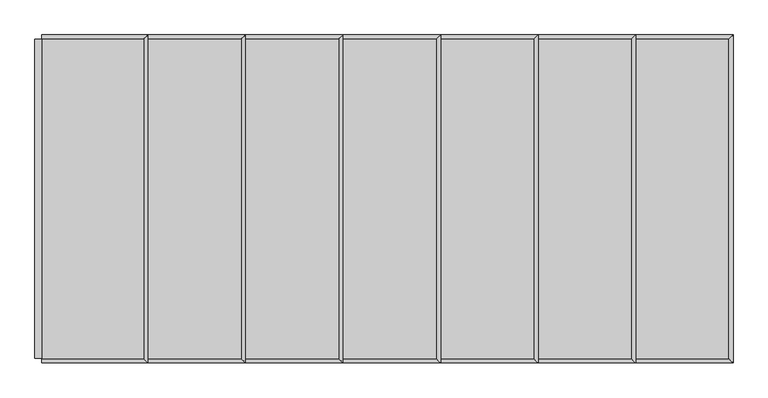
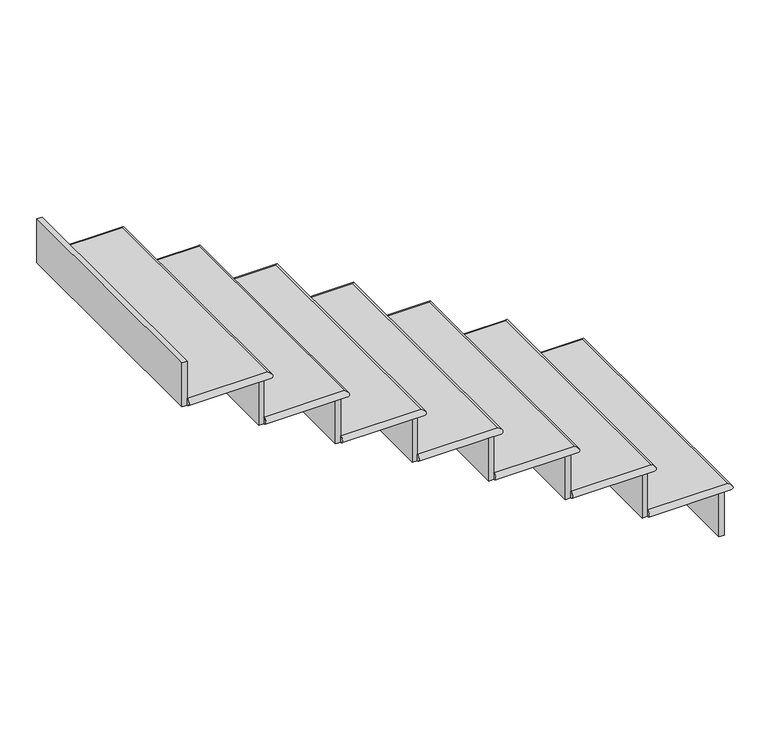
"""IFC4 building model written with IfcOpenShell, lengths in millimetres: stair flight geometry."""

from ifc_helpers import new_model, si_unit, frame, origin, place, context, project, spatial, circle_curve, ellipse_curve, faceted_brep, source, transform, mapped, element, save
from ifc_brep_helpers import plane_surface, cylinder_surface, advanced_brep


def stair_flight_95013a93(model_context):
    return source(origin(), model_context, "Body", "SolidModel", [
        advanced_brep(
        [(-8101.4581077, -7447.633999, 1837.2666667), (-8101.4581077, -7447.633999, 1862.6666667), (-8101.4581077, -8362.033999, 1862.6666667), (-8101.4581077, -8362.033999, 1837.2666667), (-8393.5581077, -7447.633999, 1862.6666667), (-8393.5581077, -8362.033999, 1862.6666667), (-8393.5581077, -8362.033999, 1837.2666667), (-8393.5581077, -7447.633999, 1837.2666667)],
        [
            (0, 1, ellipse_curve(frame((-8101.4581077, -7447.633999, 1849.9666667), z_axis=(0.7071067811865464, -0.7071067811865487, 0.0), x_axis=(0.7071067811865487, 0.7071067811865464, 0.0)), 17.9605122, 12.7)),
            (1, 2),
            (2, 3, ellipse_curve(frame((-8101.4581077, -8362.033999, 1849.9666667), z_axis=(0.7071067811865487, 0.7071067811865464, 0.0), x_axis=(-0.7071067811865464, 0.7071067811865487, 0.0)), 17.9605122, 12.7)),
            (3, 0),
            (4, 5),
            (5, 2),
            (1, 4),
            (6, 7),
            (7, 0),
            (3, 6),
            (4, 7, circle_curve(frame((-8393.5581077, -7447.633999, 1849.9666667), z_axis=(-1.0, 0.0, 0.0), x_axis=(0.0, -1.0, 0.0)), 12.7)),
            (6, 5, circle_curve(frame((-8393.5581077, -8362.033999, 1849.9666667), z_axis=(-1.0, 0.0, 0.0), x_axis=(0.0, 1.0, 0.0)), 12.7)),
        ],
        [
            cylinder_surface(frame((-8101.4581077, -7447.633999, 1849.9666667), z_axis=(0.0, 1.0, 0.0), x_axis=(-1.0, 0.0, 0.0)), 12.7),
            plane_surface(frame((-8088.7581077, -8362.033999, 1862.6666667), z_axis=(0.0, 0.0, 1.0), x_axis=(1.0, 0.0, 0.0))),
            plane_surface(frame((-8088.7581077, -8362.033999, 1837.2666667), z_axis=(0.0, 0.0, -1.0), x_axis=(-1.0, 0.0, 0.0))),
            plane_surface(frame((-8393.5581077, -7447.633999, 1862.6666667), z_axis=(-1.0, 0.0, 0.0), x_axis=(0.0, 0.0, -1.0))),
            cylinder_surface(frame((-8393.5581077, -7447.633999, 1849.9666667), z_axis=(-1.0, 0.0, 0.0), x_axis=(0.0, -1.0, 0.0)), 12.7),
            cylinder_surface(frame((-8101.4581077, -8362.033999, 1849.9666667), z_axis=(1.0, 0.0, 0.0), x_axis=(0.0, 1.0, 0.0)), 12.7),
        ],
        [
            (0, [[1, 2, 3, 4]]),
            (1, [[5, 6, -2, 7]]),
            (2, [[8, 9, -4, 10]]),
            (3, [[-5, 11, -8, 12]]),
            (4, [[-11, -7, -1, -9]]),
            (5, [[-3, -6, -12, -10]]),
        ],
    ),
        faceted_brep([(-8114.1581077, -7447.633999, 1837.2666667), (-8114.1581077, -7447.633999, 1667.9333333), (-8133.2081077, -7447.633999, 1667.9333333), (-8133.2081077, -7447.633999, 1837.2666667), (-8114.1581077, -8362.033999, 1837.2666667), (-8133.2081077, -8362.033999, 1837.2666667), (-8133.2081077, -8362.033999, 1667.9333333), (-8114.1581077, -8362.033999, 1667.9333333)], [[[0, 1, 2, 3]], [[4, 5, 6, 7]], [[1, 0, 4, 7]], [[2, 1, 7, 6]], [[3, 2, 6, 5]], [[0, 3, 5, 4]]]),
        faceted_brep([(-8393.5581077, -7447.633999, 2006.6), (-8393.5581077, -7447.633999, 1837.2666667), (-8412.6081077, -7447.633999, 1837.2666667), (-8412.6081077, -7447.633999, 2006.6), (-8393.5581077, -8362.033999, 2006.6), (-8412.6081077, -8362.033999, 2006.6), (-8412.6081077, -8362.033999, 1837.2666667), (-8393.5581077, -8362.033999, 1837.2666667)], [[[0, 1, 2, 3]], [[4, 5, 6, 7]], [[1, 0, 4, 7]], [[2, 1, 7, 6]], [[3, 2, 6, 5]], [[0, 3, 5, 4]]]),
        advanced_brep(
        [(-8672.9581077, -7447.633999, 2032.0), (-8672.9581077, -8362.033999, 2032.0), (-8380.8581077, -8362.033999, 2032.0), (-8380.8581077, -7447.633999, 2032.0), (-8672.9581077, -8362.033999, 2006.6), (-8672.9581077, -7447.633999, 2006.6), (-8380.8581077, -7447.633999, 2006.6), (-8380.8581077, -8362.033999, 2006.6)],
        [
            (0, 1),
            (1, 2),
            (2, 3),
            (3, 0),
            (4, 5),
            (5, 6),
            (6, 7),
            (7, 4),
            (0, 5, circle_curve(frame((-8672.9581077, -7447.633999, 2019.3), z_axis=(-1.0, 0.0, 0.0), x_axis=(0.0, -1.0, 0.0)), 12.7)),
            (4, 1, circle_curve(frame((-8672.9581077, -8362.033999, 2019.3), z_axis=(-1.0, 0.0, 0.0), x_axis=(0.0, 1.0, 0.0)), 12.7)),
            (6, 3, ellipse_curve(frame((-8380.8581077, -7447.633999, 2019.3), z_axis=(0.707106781186545, -0.7071067811865501, 0.0), x_axis=(0.70710678118655, 0.7071067811865449, 0.0)), 17.9605122, 12.7)),
            (2, 7, ellipse_curve(frame((-8380.8581077, -8362.033999, 2019.3), z_axis=(0.70710678118655, 0.7071067811865449, 0.0), x_axis=(-0.707106781186545, 0.7071067811865501, 0.0)), 17.9605122, 12.7)),
        ],
        [
            plane_surface(frame((-8088.7581077, -8362.033999, 2032.0), z_axis=(0.0, 0.0, 1.0), x_axis=(1.0, 0.0, 0.0))),
            plane_surface(frame((-8088.7581077, -8362.033999, 2006.6), z_axis=(0.0, 0.0, -1.0), x_axis=(-1.0, 0.0, 0.0))),
            plane_surface(frame((-8672.9581077, -7447.633999, 2032.0), z_axis=(-1.0, 0.0, 0.0), x_axis=(0.0, 0.0, -1.0))),
            cylinder_surface(frame((-8380.8581077, -7447.633999, 2019.3), z_axis=(0.0, 1.0, 0.0), x_axis=(-1.0, 0.0, 0.0)), 12.7),
            cylinder_surface(frame((-8672.9581077, -7447.633999, 2019.3), z_axis=(-1.0, 0.0, 0.0), x_axis=(0.0, -1.0, 0.0)), 12.7),
            cylinder_surface(frame((-8380.8581077, -8362.033999, 2019.3), z_axis=(1.0, 0.0, 0.0), x_axis=(0.0, 1.0, 0.0)), 12.7),
        ],
        [
            (0, [[1, 2, 3, 4]]),
            (1, [[5, 6, 7, 8]]),
            (2, [[-1, 9, -5, 10]]),
            (3, [[11, -3, 12, -7]]),
            (4, [[-9, -4, -11, -6]]),
            (5, [[-12, -2, -10, -8]]),
        ],
    ),
        faceted_brep([(-8672.9581077, -7447.633999, 2175.9333333), (-8672.9581077, -7447.633999, 2006.6), (-8692.0081077, -7447.633999, 2006.6), (-8692.0081077, -7447.633999, 2175.9333333), (-8672.9581077, -8362.033999, 2175.9333333), (-8692.0081077, -8362.033999, 2175.9333333), (-8692.0081077, -8362.033999, 2006.6), (-8672.9581077, -8362.033999, 2006.6)], [[[0, 1, 2, 3]], [[4, 5, 6, 7]], [[1, 0, 4, 7]], [[2, 1, 7, 6]], [[3, 2, 6, 5]], [[0, 3, 5, 4]]]),
        advanced_brep(
        [(-8952.3581077, -7447.633999, 2201.3333333), (-8952.3581077, -8362.033999, 2201.3333333), (-8660.2581077, -8362.033999, 2201.3333333), (-8660.2581077, -7447.633999, 2201.3333333), (-8952.3581077, -8362.033999, 2175.9333333), (-8952.3581077, -7447.633999, 2175.9333333), (-8660.2581077, -7447.633999, 2175.9333333), (-8660.2581077, -8362.033999, 2175.9333333)],
        [
            (0, 1),
            (1, 2),
            (2, 3),
            (3, 0),
            (4, 5),
            (5, 6),
            (6, 7),
            (7, 4),
            (0, 5, circle_curve(frame((-8952.3581077, -7447.633999, 2188.6333333), z_axis=(-1.0, 0.0, 0.0), x_axis=(0.0, -1.0, 0.0)), 12.7)),
            (4, 1, circle_curve(frame((-8952.3581077, -8362.033999, 2188.6333333), z_axis=(-1.0, 0.0, 0.0), x_axis=(0.0, 1.0, 0.0)), 12.7)),
            (6, 3, ellipse_curve(frame((-8660.2581077, -7447.633999, 2188.6333333), z_axis=(0.707106781186545, -0.7071067811865501, 0.0), x_axis=(0.70710678118655, 0.7071067811865449, 0.0)), 17.9605122, 12.7)),
            (2, 7, ellipse_curve(frame((-8660.2581077, -8362.033999, 2188.6333333), z_axis=(0.70710678118655, 0.7071067811865449, 0.0), x_axis=(-0.707106781186545, 0.7071067811865501, 0.0)), 17.9605122, 12.7)),
        ],
        [
            plane_surface(frame((-8368.1581077, -8362.033999, 2201.3333333), z_axis=(0.0, 0.0, 1.0), x_axis=(1.0, 0.0, 0.0))),
            plane_surface(frame((-8368.1581077, -8362.033999, 2175.9333333), z_axis=(0.0, 0.0, -1.0), x_axis=(-1.0, 0.0, 0.0))),
            plane_surface(frame((-8952.3581077, -7447.633999, 2201.3333333), z_axis=(-1.0, 0.0, 0.0), x_axis=(0.0, 0.0, -1.0))),
            cylinder_surface(frame((-8660.2581077, -7447.633999, 2188.6333333), z_axis=(0.0, 1.0, 0.0), x_axis=(-1.0, 0.0, 0.0)), 12.7),
            cylinder_surface(frame((-8952.3581077, -7447.633999, 2188.6333333), z_axis=(-1.0, 0.0, 0.0), x_axis=(0.0, -1.0, 0.0)), 12.7),
            cylinder_surface(frame((-8660.2581077, -8362.033999, 2188.6333333), z_axis=(1.0, 0.0, 0.0), x_axis=(0.0, 1.0, 0.0)), 12.7),
        ],
        [
            (0, [[1, 2, 3, 4]]),
            (1, [[5, 6, 7, 8]]),
            (2, [[-1, 9, -5, 10]]),
            (3, [[11, -3, 12, -7]]),
            (4, [[-9, -4, -11, -6]]),
            (5, [[-12, -2, -10, -8]]),
        ],
    ),
        faceted_brep([(-8952.3581077, -7447.633999, 2345.2666667), (-8952.3581077, -7447.633999, 2175.9333333), (-8971.4081077, -7447.633999, 2175.9333333), (-8971.4081077, -7447.633999, 2345.2666667), (-8952.3581077, -8362.033999, 2345.2666667), (-8971.4081077, -8362.033999, 2345.2666667), (-8971.4081077, -8362.033999, 2175.9333333), (-8952.3581077, -8362.033999, 2175.9333333)], [[[0, 1, 2, 3]], [[4, 5, 6, 7]], [[1, 0, 4, 7]], [[2, 1, 7, 6]], [[3, 2, 6, 5]], [[0, 3, 5, 4]]]),
        advanced_brep(
        [(-9231.7581077, -7447.633999, 2370.6666667), (-9231.7581077, -8362.033999, 2370.6666667), (-8939.6581077, -8362.033999, 2370.6666667), (-8939.6581077, -7447.633999, 2370.6666667), (-9231.7581077, -8362.033999, 2345.2666667), (-9231.7581077, -7447.633999, 2345.2666667), (-8939.6581077, -7447.633999, 2345.2666667), (-8939.6581077, -8362.033999, 2345.2666667)],
        [
            (0, 1),
            (1, 2),
            (2, 3),
            (3, 0),
            (4, 5),
            (5, 6),
            (6, 7),
            (7, 4),
            (0, 5, circle_curve(frame((-9231.7581077, -7447.633999, 2357.9666667), z_axis=(-1.0, 0.0, 0.0), x_axis=(0.0, -1.0, 0.0)), 12.7)),
            (4, 1, circle_curve(frame((-9231.7581077, -8362.033999, 2357.9666667), z_axis=(-1.0, 0.0, 0.0), x_axis=(0.0, 1.0, 0.0)), 12.7)),
            (6, 3, ellipse_curve(frame((-8939.6581077, -7447.633999, 2357.9666667), z_axis=(0.707106781186545, -0.7071067811865501, 0.0), x_axis=(0.70710678118655, 0.7071067811865449, 0.0)), 17.9605122, 12.7)),
            (2, 7, ellipse_curve(frame((-8939.6581077, -8362.033999, 2357.9666667), z_axis=(0.70710678118655, 0.7071067811865449, 0.0), x_axis=(-0.707106781186545, 0.7071067811865501, 0.0)), 17.9605122, 12.7)),
        ],
        [
            plane_surface(frame((-8647.5581077, -8362.033999, 2370.6666667), z_axis=(0.0, 0.0, 1.0), x_axis=(1.0, 0.0, 0.0))),
            plane_surface(frame((-8647.5581077, -8362.033999, 2345.2666667), z_axis=(0.0, 0.0, -1.0), x_axis=(-1.0, 0.0, 0.0))),
            plane_surface(frame((-9231.7581077, -7447.633999, 2370.6666667), z_axis=(-1.0, 0.0, 0.0), x_axis=(0.0, 0.0, -1.0))),
            cylinder_surface(frame((-8939.6581077, -7447.633999, 2357.9666667), z_axis=(0.0, 1.0, 0.0), x_axis=(-1.0, 0.0, 0.0)), 12.7),
            cylinder_surface(frame((-9231.7581077, -7447.633999, 2357.9666667), z_axis=(-1.0, 0.0, 0.0), x_axis=(0.0, -1.0, 0.0)), 12.7),
            cylinder_surface(frame((-8939.6581077, -8362.033999, 2357.9666667), z_axis=(1.0, 0.0, 0.0), x_axis=(0.0, 1.0, 0.0)), 12.7),
        ],
        [
            (0, [[1, 2, 3, 4]]),
            (1, [[5, 6, 7, 8]]),
            (2, [[-1, 9, -5, 10]]),
            (3, [[11, -3, 12, -7]]),
            (4, [[-9, -4, -11, -6]]),
            (5, [[-12, -2, -10, -8]]),
        ],
    ),
        faceted_brep([(-9231.7581077, -7447.633999, 2514.6), (-9231.7581077, -7447.633999, 2345.2666667), (-9250.8081077, -7447.633999, 2345.2666667), (-9250.8081077, -7447.633999, 2514.6), (-9231.7581077, -8362.033999, 2514.6), (-9250.8081077, -8362.033999, 2514.6), (-9250.8081077, -8362.033999, 2345.2666667), (-9231.7581077, -8362.033999, 2345.2666667)], [[[0, 1, 2, 3]], [[4, 5, 6, 7]], [[1, 0, 4, 7]], [[2, 1, 7, 6]], [[3, 2, 6, 5]], [[0, 3, 5, 4]]]),
        advanced_brep(
        [(-9511.1581077, -7447.633999, 2540.0), (-9511.1581077, -8362.033999, 2540.0), (-9219.0581077, -8362.033999, 2540.0), (-9219.0581077, -7447.633999, 2540.0), (-9511.1581077, -8362.033999, 2514.6), (-9511.1581077, -7447.633999, 2514.6), (-9219.0581077, -7447.633999, 2514.6), (-9219.0581077, -8362.033999, 2514.6)],
        [
            (0, 1),
            (1, 2),
            (2, 3),
            (3, 0),
            (4, 5),
            (5, 6),
            (6, 7),
            (7, 4),
            (0, 5, circle_curve(frame((-9511.1581077, -7447.633999, 2527.3), z_axis=(-1.0, 0.0, 0.0), x_axis=(0.0, -1.0, 0.0)), 12.7)),
            (4, 1, circle_curve(frame((-9511.1581077, -8362.033999, 2527.3), z_axis=(-1.0, 0.0, 0.0), x_axis=(0.0, 1.0, 0.0)), 12.7)),
            (6, 3, ellipse_curve(frame((-9219.0581077, -7447.633999, 2527.3), z_axis=(0.707106781186545, -0.7071067811865501, 0.0), x_axis=(0.70710678118655, 0.7071067811865449, 0.0)), 17.9605122, 12.7)),
            (2, 7, ellipse_curve(frame((-9219.0581077, -8362.033999, 2527.3), z_axis=(0.70710678118655, 0.7071067811865449, 0.0), x_axis=(-0.707106781186545, 0.7071067811865501, 0.0)), 17.9605122, 12.7)),
        ],
        [
            plane_surface(frame((-8926.9581077, -8362.033999, 2540.0), z_axis=(0.0, 0.0, 1.0), x_axis=(1.0, 0.0, 0.0))),
            plane_surface(frame((-8926.9581077, -8362.033999, 2514.6), z_axis=(0.0, 0.0, -1.0), x_axis=(-1.0, 0.0, 0.0))),
            plane_surface(frame((-9511.1581077, -7447.633999, 2540.0), z_axis=(-1.0, 0.0, 0.0), x_axis=(0.0, 0.0, -1.0))),
            cylinder_surface(frame((-9219.0581077, -7447.633999, 2527.3), z_axis=(0.0, 1.0, 0.0), x_axis=(-1.0, 0.0, 0.0)), 12.7),
            cylinder_surface(frame((-9511.1581077, -7447.633999, 2527.3), z_axis=(-1.0, 0.0, 0.0), x_axis=(0.0, -1.0, 0.0)), 12.7),
            cylinder_surface(frame((-9219.0581077, -8362.033999, 2527.3), z_axis=(1.0, 0.0, 0.0), x_axis=(0.0, 1.0, 0.0)), 12.7),
        ],
        [
            (0, [[1, 2, 3, 4]]),
            (1, [[5, 6, 7, 8]]),
            (2, [[-1, 9, -5, 10]]),
            (3, [[11, -3, 12, -7]]),
            (4, [[-9, -4, -11, -6]]),
            (5, [[-12, -2, -10, -8]]),
        ],
    ),
        faceted_brep([(-9511.1581077, -7447.633999, 2683.9333333), (-9511.1581077, -7447.633999, 2514.6), (-9530.2081077, -7447.633999, 2514.6), (-9530.2081077, -7447.633999, 2683.9333333), (-9511.1581077, -8362.033999, 2683.9333333), (-9530.2081077, -8362.033999, 2683.9333333), (-9530.2081077, -8362.033999, 2514.6), (-9511.1581077, -8362.033999, 2514.6)], [[[0, 1, 2, 3]], [[4, 5, 6, 7]], [[1, 0, 4, 7]], [[2, 1, 7, 6]], [[3, 2, 6, 5]], [[0, 3, 5, 4]]]),
        advanced_brep(
        [(-9790.5581077, -7447.633999, 2709.3333333), (-9790.5581077, -8362.033999, 2709.3333333), (-9498.4581077, -8362.033999, 2709.3333333), (-9498.4581077, -7447.633999, 2709.3333333), (-9790.5581077, -8362.033999, 2683.9333333), (-9790.5581077, -7447.633999, 2683.9333333), (-9498.4581077, -7447.633999, 2683.9333333), (-9498.4581077, -8362.033999, 2683.9333333)],
        [
            (0, 1),
            (1, 2),
            (2, 3),
            (3, 0),
            (4, 5),
            (5, 6),
            (6, 7),
            (7, 4),
            (0, 5, circle_curve(frame((-9790.5581077, -7447.633999, 2696.6333333), z_axis=(-1.0, 0.0, 0.0), x_axis=(0.0, -1.0, 0.0)), 12.7)),
            (4, 1, circle_curve(frame((-9790.5581077, -8362.033999, 2696.6333333), z_axis=(-1.0, 0.0, 0.0), x_axis=(0.0, 1.0, 0.0)), 12.7)),
            (6, 3, ellipse_curve(frame((-9498.4581077, -7447.633999, 2696.6333333), z_axis=(0.707106781186545, -0.7071067811865501, 0.0), x_axis=(0.70710678118655, 0.7071067811865449, 0.0)), 17.9605122, 12.7)),
            (2, 7, ellipse_curve(frame((-9498.4581077, -8362.033999, 2696.6333333), z_axis=(0.70710678118655, 0.7071067811865449, 0.0), x_axis=(-0.707106781186545, 0.7071067811865501, 0.0)), 17.9605122, 12.7)),
        ],
        [
            plane_surface(frame((-9206.3581077, -8362.033999, 2709.3333333), z_axis=(0.0, 0.0, 1.0), x_axis=(1.0, 0.0, 0.0))),
            plane_surface(frame((-9206.3581077, -8362.033999, 2683.9333333), z_axis=(0.0, 0.0, -1.0), x_axis=(-1.0, 0.0, 0.0))),
            plane_surface(frame((-9790.5581077, -7447.633999, 2709.3333333), z_axis=(-1.0, 0.0, 0.0), x_axis=(0.0, 0.0, -1.0))),
            cylinder_surface(frame((-9498.4581077, -7447.633999, 2696.6333333), z_axis=(0.0, 1.0, 0.0), x_axis=(-1.0, 0.0, 0.0)), 12.7),
            cylinder_surface(frame((-9790.5581077, -7447.633999, 2696.6333333), z_axis=(-1.0, 0.0, 0.0), x_axis=(0.0, -1.0, 0.0)), 12.7),
            cylinder_surface(frame((-9498.4581077, -8362.033999, 2696.6333333), z_axis=(1.0, 0.0, 0.0), x_axis=(0.0, 1.0, 0.0)), 12.7),
        ],
        [
            (0, [[1, 2, 3, 4]]),
            (1, [[5, 6, 7, 8]]),
            (2, [[-1, 9, -5, 10]]),
            (3, [[11, -3, 12, -7]]),
            (4, [[-9, -4, -11, -6]]),
            (5, [[-12, -2, -10, -8]]),
        ],
    ),
        faceted_brep([(-9790.5581077, -7447.633999, 2853.2666667), (-9790.5581077, -7447.633999, 2683.9333333), (-9809.6081077, -7447.633999, 2683.9333333), (-9809.6081077, -7447.633999, 2853.2666667), (-9790.5581077, -8362.033999, 2853.2666667), (-9809.6081077, -8362.033999, 2853.2666667), (-9809.6081077, -8362.033999, 2683.9333333), (-9790.5581077, -8362.033999, 2683.9333333)], [[[0, 1, 2, 3]], [[4, 5, 6, 7]], [[1, 0, 4, 7]], [[2, 1, 7, 6]], [[3, 2, 6, 5]], [[0, 3, 5, 4]]]),
        faceted_brep([(-10069.9581077, -7447.633999, 3022.6), (-10069.9581077, -7447.633999, 2853.2666667), (-10089.0081077, -7447.633999, 2853.2666667), (-10089.0081077, -7447.633999, 3022.6), (-10069.9581077, -8362.033999, 3022.6), (-10089.0081077, -8362.033999, 3022.6), (-10089.0081077, -8362.033999, 2853.2666667), (-10069.9581077, -8362.033999, 2853.2666667)], [[[0, 1, 2, 3]], [[4, 5, 6, 7]], [[1, 0, 4, 7]], [[2, 1, 7, 6]], [[3, 2, 6, 5]], [[0, 3, 5, 4]]]),
        advanced_brep(
        [(-10069.9581077, -7447.633999, 2878.6666667), (-10069.9581077, -8362.033999, 2878.6666667), (-9777.8581077, -8362.033999, 2878.6666667), (-9777.8581077, -7447.633999, 2878.6666667), (-10069.9581077, -8362.033999, 2853.2666667), (-10069.9581077, -7447.633999, 2853.2666667), (-9777.8581077, -7447.633999, 2853.2666667), (-9777.8581077, -8362.033999, 2853.2666667)],
        [
            (0, 1),
            (1, 2),
            (2, 3),
            (3, 0),
            (4, 5),
            (5, 6),
            (6, 7),
            (7, 4),
            (0, 5, circle_curve(frame((-10069.9581077, -7447.633999, 2865.9666667), z_axis=(-1.0, 0.0, 0.0), x_axis=(0.0, -1.0, 0.0)), 12.7)),
            (4, 1, circle_curve(frame((-10069.9581077, -8362.033999, 2865.9666667), z_axis=(-1.0, 0.0, 0.0), x_axis=(0.0, 1.0, 0.0)), 12.7)),
            (6, 3, ellipse_curve(frame((-9777.8581077, -7447.633999, 2865.9666667), z_axis=(0.707106781186545, -0.7071067811865501, 0.0), x_axis=(0.70710678118655, 0.7071067811865449, 0.0)), 17.9605122, 12.7)),
            (2, 7, ellipse_curve(frame((-9777.8581077, -8362.033999, 2865.9666667), z_axis=(0.70710678118655, 0.7071067811865449, 0.0), x_axis=(-0.707106781186545, 0.7071067811865501, 0.0)), 17.9605122, 12.7)),
        ],
        [
            plane_surface(frame((-9485.7581077, -8362.033999, 2878.6666667), z_axis=(0.0, 0.0, 1.0), x_axis=(1.0, 0.0, 0.0))),
            plane_surface(frame((-9485.7581077, -8362.033999, 2853.2666667), z_axis=(0.0, 0.0, -1.0), x_axis=(-1.0, 0.0, 0.0))),
            plane_surface(frame((-10069.9581077, -7447.633999, 2878.6666667), z_axis=(-1.0, 0.0, 0.0), x_axis=(0.0, 0.0, -1.0))),
            cylinder_surface(frame((-9777.8581077, -7447.633999, 2865.9666667), z_axis=(0.0, 1.0, 0.0), x_axis=(-1.0, 0.0, 0.0)), 12.7),
            cylinder_surface(frame((-10069.9581077, -7447.633999, 2865.9666667), z_axis=(-1.0, 0.0, 0.0), x_axis=(0.0, -1.0, 0.0)), 12.7),
            cylinder_surface(frame((-9777.8581077, -8362.033999, 2865.9666667), z_axis=(1.0, 0.0, 0.0), x_axis=(0.0, 1.0, 0.0)), 12.7),
        ],
        [
            (0, [[1, 2, 3, 4]]),
            (1, [[5, 6, 7, 8]]),
            (2, [[-1, 9, -5, 10]]),
            (3, [[11, -3, 12, -7]]),
            (4, [[-9, -4, -11, -6]]),
            (5, [[-12, -2, -10, -8]]),
        ],
    ),
    ])


if __name__ == "__main__":
    model = new_model("IFC4")
    model_context = context("Model", 3, world=origin())
    ifc_project = project(units=[si_unit("LENGTHUNIT", "METRE", prefix="MILLI")], contexts=[model_context])
    site = spatial("IfcSite", under=ifc_project)
    building = spatial("IfcBuilding", under=site)
    placement = place(None, origin())
    stair_flight_shape = stair_flight_95013a93(model_context)
    element("IfcStairFlight", 1, at=placement, inside=building, context=model_context, shape_type="MappedRepresentation", body=[
        mapped(stair_flight_shape, transform((0.0, 0.0, 0.0), x_axis=(1.0, 0.0, 0.0), y_axis=(0.0, 1.0, 0.0), z_axis=(0.0, 0.0, 1.0))),
    ])
    save(model, "model.ifc")

# Revit data of these elements
# Element 1 (IfcStairFlight)
#   Materials on its faces: "Wood - Cherry"
# Materials
#   "Wood - Cherry": class "Unassigned", colour RGB 226 177 128, transparency 0
